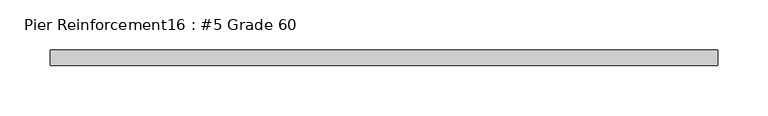
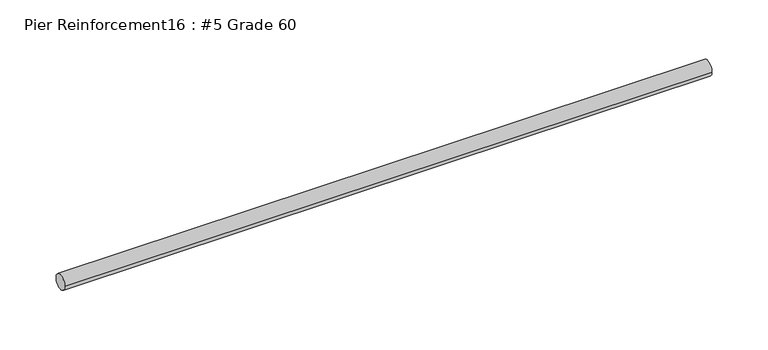
"""IFC4 building model written with IfcOpenShell, lengths in millimetres: proxy geometry, Pier Reinforcement16 : #5 Grade 60."""

from ifc_helpers import new_model, si_unit, point, frame, frame_2d, origin, place, context, project, spatial, circle_curve, trimmed, segment, composite_curve, outline, extrude, source, transform, mapped, element, save


def pier_reinforcement16_5_grade_60_c3fb3d78(model_context):
    return source(origin(), model_context, "Body", "SweptSolid", [
        extrude(outline(composite_curve([segment(trimmed(circle_curve(frame_2d((-536315.9913841, -55.5625)), 7.9375), [point((-536308.0538841, -55.5625))], [point((-536323.9288841, -55.5625))], False, "CARTESIAN"), True, "CONTINUOUS"), segment(trimmed(circle_curve(frame_2d((-536315.9913841, -55.5625)), 7.9375), [point((-536323.9288841, -55.5625))], [point((-536308.0538841, -55.5625))], False, "CARTESIAN"), True, "CONTINUOUS")], self_intersect=False)), frame((589567.2422365, 0.0, 0.0), z_axis=(1.0, 0.0, 0.0), x_axis=(0.0, 1.0, 0.0)), (0.0, 0.0, 1.0), 666.75),
    ])


if __name__ == "__main__":
    model = new_model("IFC4")
    model_context = context("Model", 3, world=origin())
    ifc_project = project(units=[si_unit("LENGTHUNIT", "METRE", prefix="MILLI")], contexts=[model_context])
    site = spatial("IfcSite", under=ifc_project)
    building = spatial("IfcBuilding", under=site)
    placement = place(None, origin())
    pier_reinforcement16_5_grade_60_shape = pier_reinforcement16_5_grade_60_c3fb3d78(model_context)
    element("IfcBuildingElementProxy", 1, Name="Pier Reinforcement16 : #5 Grade 60", ObjectType="Pier Reinforcement16 : #5 Grade 60", at=placement, inside=building, context=model_context, shape_type="MappedRepresentation", body=[
        mapped(pier_reinforcement16_5_grade_60_shape, transform((0.0, 0.0, 0.0), x_axis=(1.0, 0.0, 0.0), y_axis=(0.0, 1.0, 0.0), z_axis=(0.0, 0.0, 1.0))),
    ])
    save(model, "model.ifc")

# Revit data of these elements
# Element 1 (IfcBuildingElementProxy, "Pier Reinforcement16 : #5 Grade 60")
#   Materials on its faces: "#4 GR. 60 REINF. @ 16\" O.C. EW."
# Materials
#   "#4 GR. 60 REINF. @ 16\" O.C. EW.": class "Generic", colour RGB 84 83 81, transparency 0, Cost = 0
